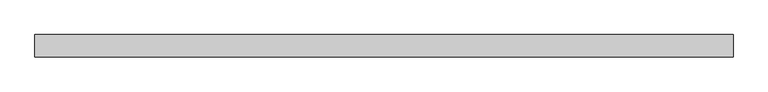
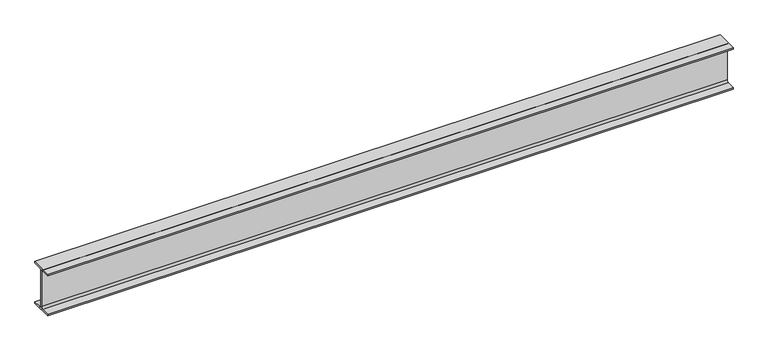
"""IFC4 building model written with IfcOpenShell, lengths in millimetres: beam geometry, 0912_Steel Framing_H-KSD3502 : H_SB_ASB_H-250x125x6x9."""

from ifc_helpers import new_model, si_unit, point, frame, frame_2d, origin, place, context, project, spatial, polyline, circle_curve, trimmed, segment, composite_curve, outline, extrude, source, transform, mapped, element, save


def beam_63befc3e(model_context):
    return source(origin(), model_context, "Body", "SweptSolid", [
        extrude(outline(composite_curve([segment(polyline([(62.5, -116.0), (62.5, -125.0), (-62.5, -125.0), (-62.5, -116.0), (-15.0, -116.0)]), True, "CONTINUOUS"), segment(trimmed(circle_curve(frame_2d((-15.0, -104.0)), 12.0), [point((-15.0, -116.0))], [point((-3.0, -104.0))], True, "CARTESIAN"), True, "CONTINUOUS"), segment(polyline([(-3.0, -104.0), (-3.0, 104.0)]), True, "CONTINUOUS"), segment(trimmed(circle_curve(frame_2d((-15.0, 104.0)), 12.0), [point((-3.0, 104.0))], [point((-15.0, 116.0))], True, "CARTESIAN"), True, "CONTINUOUS"), segment(polyline([(-15.0, 116.0), (-62.5, 116.0), (-62.5, 125.0), (62.5, 125.0), (62.5, 116.0), (15.0, 116.0)]), True, "CONTINUOUS"), segment(trimmed(circle_curve(frame_2d((15.0, 104.0)), 12.0), [point((15.0, 116.0))], [point((3.0, 104.0))], True, "CARTESIAN"), True, "CONTINUOUS"), segment(polyline([(3.0, 104.0), (3.0, -104.0)]), True, "CONTINUOUS"), segment(trimmed(circle_curve(frame_2d((15.0, -104.0)), 12.0), [point((3.0, -104.0))], [point((15.0, -116.0))], True, "CARTESIAN"), True, "CONTINUOUS"), segment(polyline([(15.0, -116.0), (62.5, -116.0)]), True, "CONTINUOUS")], self_intersect=False)), frame((-1987.2999994, 0.0, 0.0), z_axis=(1.0, 0.0, 0.0), x_axis=(0.0, 1.0, 0.0)), (0.0, 0.0, 1.0), 3892.0999994),
    ])


if __name__ == "__main__":
    model = new_model("IFC4")
    model_context = context("Model", 3, world=origin())
    ifc_project = project(units=[si_unit("LENGTHUNIT", "METRE", prefix="MILLI")], contexts=[model_context])
    site = spatial("IfcSite", under=ifc_project)
    building = spatial("IfcBuilding", under=site)
    placement = place(None, origin())
    beam_shape = beam_63befc3e(model_context)
    element("IfcBeam", 1, ObjectType="0912_Steel Framing_H-KSD3502 : H_SB_ASB_H-250x125x6x9", at=placement, inside=building, context=model_context, shape_type="MappedRepresentation", body=[
        mapped(beam_shape, transform((0.0, 0.0, 0.0), x_axis=(1.0, 0.0, 0.0), y_axis=(0.0, 1.0, 0.0), z_axis=(0.0, 0.0, 1.0))),
    ])
    save(model, "model.ifc")

# Revit data of these elements
# Type "0912_Steel Framing_H-KSD3502 : H_SB_ASB_H-250x125x6x9"
#   H_WM Code_1 = "S01AA003-00001 | Main Steel Structure Fabrication Work | Shelter/Building | Light Steel - Standard (30KG/M>Weight) | Material: (   )"
#   H_WM Code_2 = "S03AA029-00001 | Main Steel Structure Erection Work | Shelter/Building | Light Steel (30KG/M>Weight) | Material: (   )"
#   H_WM Code_3 = "S01AA010-00001 | Main Steel Structure Fabrication Work | Shelter/Building | Steel Painting/Coating | for Non-Fireproofed Steel Surface, Surface Preparation, Primer, Second & Final Coat | Material: (   )"
#   H_Q'ty Cal Type Tag = "SB-Q2"
#   Width = 12.5 cm
#   Web Thickness = 0.6 cm
#   Web Fillet = 1.2 cm
#   Warping Constant = 42539.8 cm⁶
#   W = 0
#   Torsional Moment of Inertia = 7.8102 cm⁴
#   Section Area = 37.66 cm²
#   Plastic Modulus weak axis = 73.1 cm³
#   Plastic Modulus strong axis = 366.0 cm³
#   Perimeter = 0.97 m²/m
#   Nominal Weight = 29.60 kgf/m
#   Moment of Inertia weak axis = 294.00 cm⁴
#   Moment of Inertia strong axis = 4050.00 cm⁴
#   Height = 25.0 cm
#   Flange Thickness = 0.9 cm
#   Elastic Modulus weak axis = 47.0 cm³
#   Elastic Modulus strong axis = 324.0 cm³
#   Centroid Vertical = 12.5 cm
#   Centroid Horizontal = 6.25 cm
#   Ix = 40500000
#   Length [instance default] = 1.5240 m
#   Zx = 366000
#   b = 0.1250 m
#   h = 0.2500 m
#   r = 0.0120 m
#   s = 0.0060 m
#   t = 0.0090 m
#   A = 0.003766 m²
#   Structural Material [instance default] = Steel, 45-345
#   Assembly Code = ""
# Element 1 (IfcBeam, "0912_Steel Framing_H-KSD3502 : H_SB_ASB_H-250x125x6x9")
#   Structural Material = none
# Materials
#   "Steel, 45-345": class "Metal", colour RGB 189 187 185, transparency 0, Description = "Steel 345 MPa", Cost = 0
